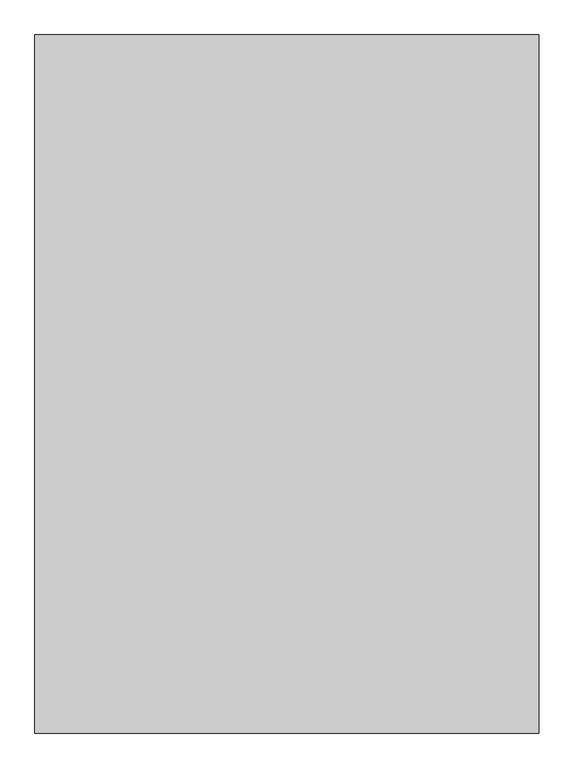
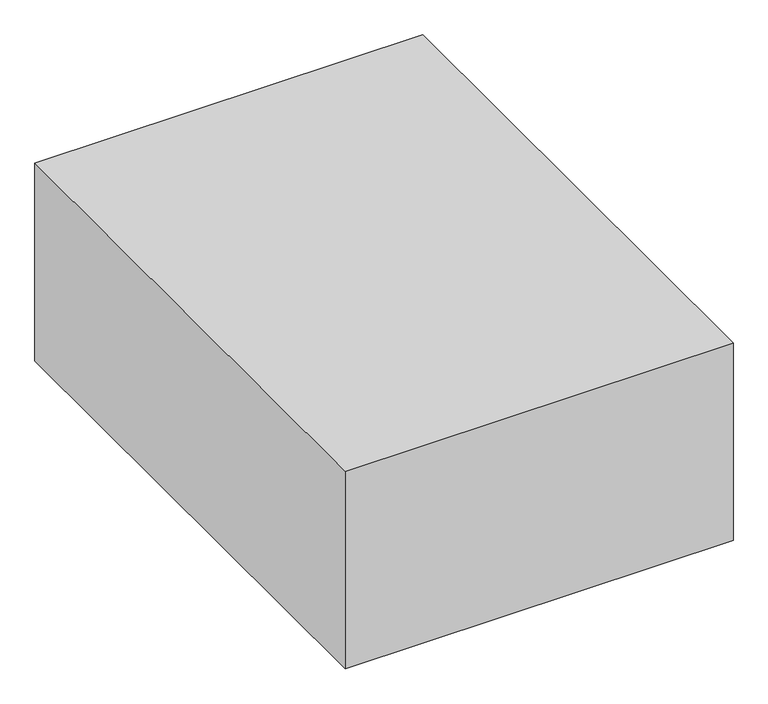
"""IFC4 building model written with IfcOpenShell, lengths in millimetres: proxy geometry, Space Planning Box_hec : Space Planning Box_hec."""

from ifc_helpers import new_model, si_unit, origin, origin_with_axes, place, context, project, spatial, polyline, outline, extrude, source, transform, mapped, element, save


def generic_models_5926095e(model_context):
    return source(origin(), model_context, "Body", "SweptSolid", [
        extrude(outline(polyline([(3250.0, 4500.0), (3250.0, -4500.0), (-3250.0, -4500.0), (-3250.0, 4500.0), (3250.0, 4500.0)])), origin_with_axes(), (0.0, 0.0, 1.0), 3500.0),
    ])


if __name__ == "__main__":
    model = new_model("IFC4")
    model_context = context("Model", 3, world=origin())
    ifc_project = project(units=[si_unit("LENGTHUNIT", "METRE", prefix="MILLI")], contexts=[model_context])
    site = spatial("IfcSite", under=ifc_project)
    building = spatial("IfcBuilding", under=site)
    placement = place(None, origin())
    generic_models_shape = generic_models_5926095e(model_context)
    element("IfcBuildingElementProxy", 1, Name="Space Planning Box_hec : Space Planning Box_hec", ObjectType="Space Planning Box_hec : Space Planning Box_hec", at=placement, inside=building, context=model_context, shape_type="MappedRepresentation", body=[
        mapped(generic_models_shape, transform((0.0, 0.0, 0.0), x_axis=(1.0, 0.0, 0.0), y_axis=(0.0, 1.0, 0.0), z_axis=(0.0, 0.0, 1.0))),
    ])
    save(model, "model.ifc")

# Revit data of these elements
# Type "Space Planning Box_hec : Space Planning Box_hec"
#   Type Comments = "..."
#   Room Name [instance default] = "?"
#   Interior Finish [instance default] = ""
#   Exterior Finish [instance default] = ""
#   Department [instance default] = ""
#   Assembly Code = "..."
#   ceiling height [instance default] = 0
#   Width [instance default] = 1524 mm
#   Program Area [instance default] = 0.00 m²
#   Length [instance default] = 1524 mm
#   Height [instance default] = 1524 mm
#   Area [instance default] = 2.32258 m²
#   Fill Color [instance default] = Cyan
#   Default Elevation = 0
# Element 1 (IfcBuildingElementProxy, "Space Planning Box_hec : Space Planning Box_hec")
#   Room Name = "Battery Room"
#   Exterior Finish = "N/A..N/A,,EW2..N/A..N/A"
#   Department = "EL"
#   Width = 6500 mm
#   Program Area = 58.50 m²
#   Length = 9000 mm
#   Height = 3500 mm
#   Area = 58.50 m²
#   Fill Color = Orange
#   Materials on its faces: "Orange"
# Materials
#   "Cyan": class "Generic", colour RGB 0 255 255, transparency 0.2, Cost = 0
#   "Orange": class "Generic", colour RGB 255 165 0, transparency 0.2, Cost = 0
